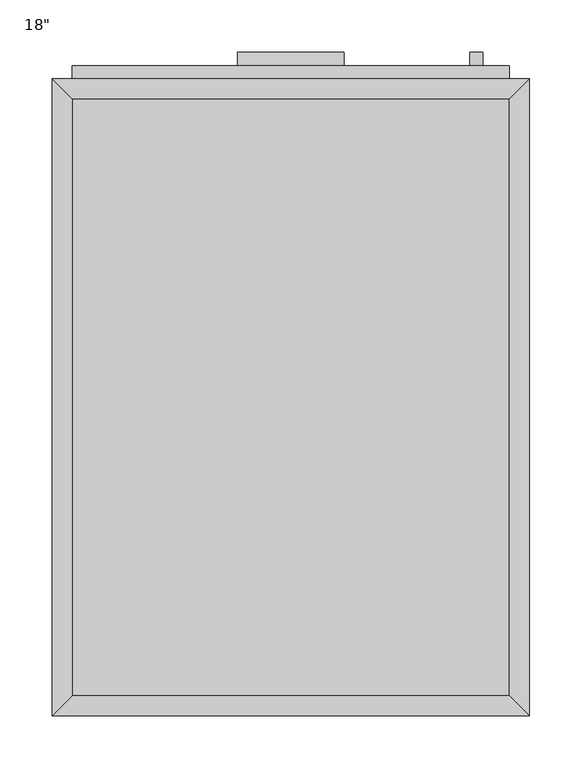
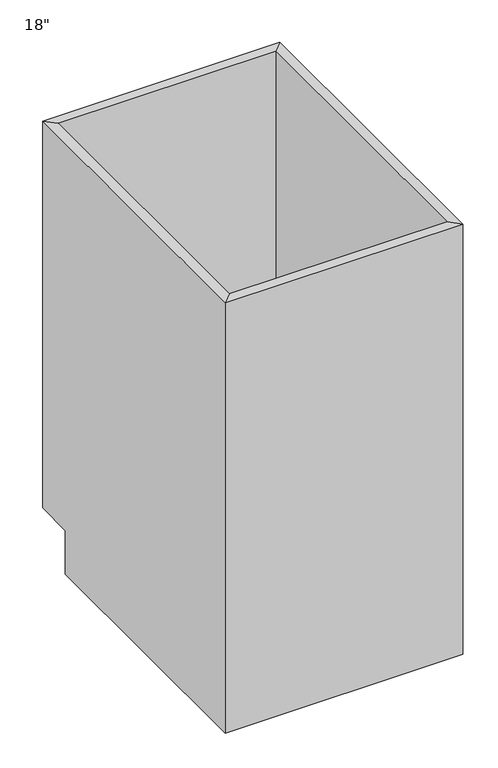
"""IFC4 building model written with IfcOpenShell, lengths in millimetres: furniture geometry."""

from ifc_helpers import new_model, si_unit, frame, origin, place, context, project, spatial, polyline, outline, extrude, faceted_brep, source, transform, mapped, element, save


def furniture_07bc9410(model_context):
    return source(origin(), model_context, "Body", "SolidModel", [
        faceted_brep([(228.2877049, 590.55, 876.3), (-190.8122951, 590.55, 876.3), (-190.8122951, 590.55, 88.9), (228.2877049, 590.55, 88.9), (247.3377049, 609.6, 876.3), (-209.8622951, 609.6, 876.3), (247.3377049, 609.6, 88.9), (-209.8622951, 609.6, 88.9), (-190.8122951, 19.05, 876.3), (-190.8122951, 19.05, 88.9), (-190.8122951, 533.4, 88.9), (-209.8622951, 0.0, 876.3), (-209.8622951, 533.4, 88.9), (-209.8622951, 533.4, 0.0), (-209.8622951, 0.0, 0.0), (228.2877049, 19.05, 876.3), (228.2877049, 19.05, 88.9), (247.3377049, 0.0, 876.3), (247.3377049, 0.0, 0.0), (228.2877049, 533.4, 88.9), (247.3377049, 533.4, 0.0), (247.3377049, 533.4, 88.9)], [[[0, 1, 2, 3]], [[0, 4, 5, 1]], [[4, 6, 7, 5]], [[2, 7, 6, 3]], [[1, 8, 9, 10, 2]], [[5, 11, 8, 1]], [[7, 12, 13, 14, 11, 5]], [[2, 10, 12, 7]], [[8, 15, 16, 9]], [[11, 17, 15, 8]], [[14, 18, 17, 11]], [[3, 19, 16, 15, 0]], [[0, 15, 17, 4]], [[4, 17, 18, 20, 21, 6]], [[6, 21, 19, 3]], [[10, 9, 16, 19]], [[18, 14, 13, 20]], [[13, 12, 10, 19, 21, 20]]]),
        extrude(outline(polyline([(202.8877049, 635.0), (202.8877049, 622.3), (190.1877049, 622.3), (190.1877049, 635.0), (202.8877049, 635.0)])), frame((0.0, 0.0, 596.9), z_axis=(0.0, 0.0, 1.0), x_axis=(1.0, 0.0, 0.0)), (0.0, 0.0, 1.0), 101.6),
        extrude(outline(polyline([(69.5377049, 635.0), (69.5377049, 622.3), (-32.0622951, 622.3), (-32.0622951, 635.0), (69.5377049, 635.0)])), frame((0.0, 0.0, 819.15), z_axis=(0.0, 0.0, 1.0), x_axis=(1.0, 0.0, 0.0)), (0.0, 0.0, 1.0), 12.7),
        extrude(outline(polyline([(228.2877049, 622.3), (228.2877049, 609.6), (-190.8122951, 609.6), (-190.8122951, 622.3), (228.2877049, 622.3)])), frame((0.0, 0.0, 107.95), z_axis=(0.0, 0.0, 1.0), x_axis=(1.0, 0.0, 0.0)), (0.0, 0.0, 1.0), 628.65),
        extrude(outline(polyline([(228.2877049, 622.3), (228.2877049, 609.6), (-190.8122951, 609.6), (-190.8122951, 622.3), (228.2877049, 622.3)])), frame((0.0, 0.0, 755.65), z_axis=(0.0, 0.0, 1.0), x_axis=(1.0, 0.0, 0.0)), (0.0, 0.0, 1.0), 101.6),
        extrude(outline(polyline([(228.2877049, 19.05), (-190.8122951, 19.05), (-190.8122951, 590.55), (228.2877049, 590.55), (228.2877049, 19.05)])), frame((0.0, 0.0, 88.9), z_axis=(0.0, 0.0, 1.0), x_axis=(1.0, 0.0, 0.0)), (0.0, 0.0, 1.0), 19.05),
    ])


if __name__ == "__main__":
    model = new_model("IFC4")
    model_context = context("Model", 3, world=origin())
    ifc_project = project(units=[si_unit("LENGTHUNIT", "METRE", prefix="MILLI")], contexts=[model_context])
    site = spatial("IfcSite", under=ifc_project)
    building = spatial("IfcBuilding", under=site)
    placement = place(None, origin())
    furniture_shape = furniture_07bc9410(model_context)
    element("IfcFurniture", 1, ObjectType="Base Cabinet-Single Door & Drawer : 18\"", at=placement, inside=building, context=model_context, shape_type="MappedRepresentation", body=[
        mapped(furniture_shape, transform((0.0, 0.0, 0.0), x_axis=(1.0, 0.0, 0.0), y_axis=(0.0, 1.0, 0.0), z_axis=(0.0, 0.0, 1.0))),
    ])
    save(model, "model.ifc")

# Revit data of these elements
# Type "Base Cabinet-Single Door & Drawer : 18\""
#   COBie.Type.CreatedBy = "doug.wood@us.ibm.com"
#   COBie.Type.CreatedOn = "2016-04-14T02:14:45"
#   COBie.Type.Name = "Casework_Base Cabinet-Single Door & Drawer_18\""
#   COBie.Type.Category = "23-40 35 17 47 11 : Kitchen Casework"
#   COBie.Type.Description = "Base Cabinet-Single Door & Drawer_18\""
#   COBie.Type.Manufacturer = ""
#   COBie.Type.ModelNumber = ""
#   Assembly Code = "C1030410"
#   COBie.Type.ReplacementCost = 0
#   Depth = 2' - 0"
#   Height = 2' - 10 1/2"
#   Toe Depth = 0' - 3"
#   Toe Height = 0' - 3 1/2"
#   Width = 1' - 6"
#   COBie.Type = no
#   Cabinet Material = none
#   Drawer Material = none
#   Handle Material = Cabinets - Handles
# Element 1 (IfcFurniture, "Base Cabinet-Single Door & Drawer : 18\"")
#   Materials on its faces: "Cabinets", "Cabinets - Handles"
# Materials
#   "Cabinets - Handles": class "Metal", colour RGB 57 57 57, transparency 0
#   "Cabinets": class "Miscellaneous", colour RGB 249 249 249, transparency 0
